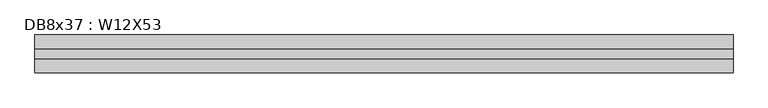
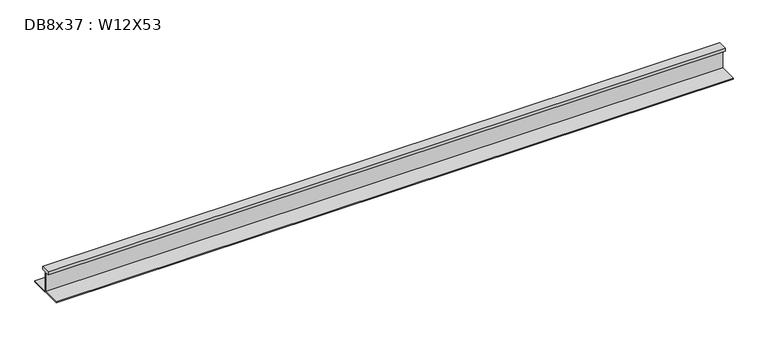
"""IFC4 building model written with IfcOpenShell, lengths in millimetres: beam geometry, DB8x37 : W12X53."""

from ifc_helpers import new_model, si_unit, frame, origin, place, context, project, spatial, polyline, outline, extrude, source, transform, mapped, element, save


def db8x37_w12x53_1dfed5d5(model_context):
    return source(origin(), model_context, "Body", "SweptSolid", [
        extrude(outline(polyline([(38.1, 145.415), (38.1, 120.015), (2.921, 120.015), (2.921, -48.4505), (152.4, -48.4505), (152.4, -58.1025), (-152.4, -58.1025), (-152.4, -48.4505), (-2.921, -48.4505), (-2.921, 120.015), (-38.1, 120.015), (-38.1, 145.415), (38.1, 145.415)])), frame((-2878.8042219, 0.0, 0.0), z_axis=(1.0, 0.0, 0.0), x_axis=(0.0, 1.0, 0.0)), (0.0, 0.0, 1.0), 5601.668375),
    ])


if __name__ == "__main__":
    model = new_model("IFC4")
    model_context = context("Model", 3, world=origin())
    ifc_project = project(units=[si_unit("LENGTHUNIT", "METRE", prefix="MILLI")], contexts=[model_context])
    site = spatial("IfcSite", under=ifc_project)
    building = spatial("IfcBuilding", under=site)
    placement = place(None, origin())
    db8x37_w12x53_shape = db8x37_w12x53_1dfed5d5(model_context)
    element("IfcBeam", 1, ObjectType="DB8x37 : W12X53", at=placement, inside=building, context=model_context, shape_type="MappedRepresentation", body=[
        mapped(db8x37_w12x53_shape, transform((0.0, 0.0, 0.0), x_axis=(1.0, 0.0, 0.0), y_axis=(0.0, 1.0, 0.0), z_axis=(0.0, 0.0, 1.0))),
    ])
    save(model, "model.ifc")

# Revit data of these elements
# Type "DB8x37 : W12X53"
#   Assembly Code = "B10"
#   W = 53
#   Length [instance default] = 5' - 0"
#   bf = 0' - 10"
#   d = 1' - 0.1"
#   k = 0' - 1 3/8"
#   k2 = 0' - 0.8"
#   tf = 0' - 0.575"
#   tw = 0' - 0.345"
#   A = 0.108333 SF
#   Structural Material [instance default] = Steel ASTM A992
# Element 1 (IfcBeam, "DB8x37 : W12X53")
#   Materials on its faces: "Steel ASTM A992"
# Materials
#   "Steel ASTM A992": class "Metal", colour RGB 199 199 199, transparency 0, Description = "Structural steel 50ksi", Cost = 0
